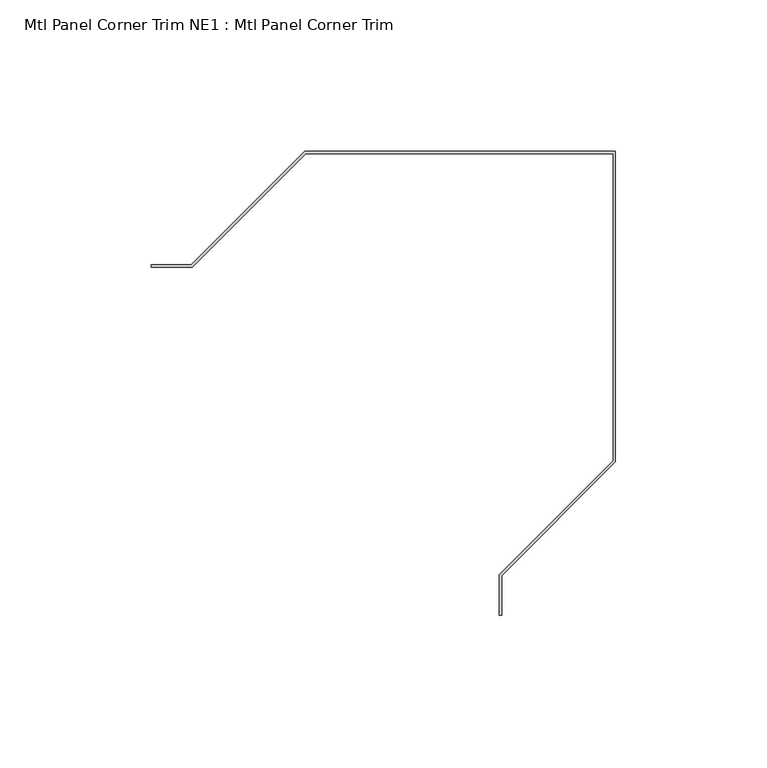
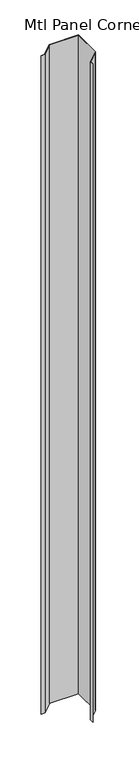
"""IFC4 building model written with IfcOpenShell, lengths in millimetres: proxy geometry, Mtl Panel Corner Trim NE1 : Mtl Panel Corner Trim."""

from ifc_helpers import new_model, si_unit, frame, origin, place, context, project, spatial, polyline, outline, extrude, source, transform, mapped, element, save


def mtl_panel_corner_trim_ne1_mtl_panel_corner_trim_1dc4974f(model_context):
    return source(origin(), model_context, "Body", "SweptSolid", [
        extrude(outline(polyline([(590354.0764739, -531753.7703841), (590354.0764739, -531740.2994038), (590391.6621239, -531702.7137538), (590391.6621239, -531601.1227341), (590290.0711042, -531601.1227341), (590252.5807042, -531638.6131341), (590239.0144739, -531638.6131341), (590239.0144739, -531637.8193841), (590252.2519222, -531637.8193841), (590289.7423222, -531600.3289841), (590392.4558739, -531600.3289841), (590392.4558739, -531703.0425358), (590354.8638739, -531740.6345358), (590354.8638739, -531753.7703841), (590354.0764739, -531753.7703841)])), frame((0.0, 0.0, 6.35), z_axis=(0.0, 0.0, 1.0), x_axis=(1.0, 0.0, 0.0)), (0.0, 0.0, 1.0), 2432.05),
    ])


if __name__ == "__main__":
    model = new_model("IFC4")
    model_context = context("Model", 3, world=origin())
    ifc_project = project(units=[si_unit("LENGTHUNIT", "METRE", prefix="MILLI")], contexts=[model_context])
    site = spatial("IfcSite", under=ifc_project)
    building = spatial("IfcBuilding", under=site)
    placement = place(None, origin())
    mtl_panel_corner_trim_ne1_mtl_panel_corner_trim_shape = mtl_panel_corner_trim_ne1_mtl_panel_corner_trim_1dc4974f(model_context)
    element("IfcBuildingElementProxy", 1, Name="Mtl Panel Corner Trim NE1 : Mtl Panel Corner Trim", ObjectType="Mtl Panel Corner Trim NE1 : Mtl Panel Corner Trim", at=placement, inside=building, context=model_context, shape_type="MappedRepresentation", body=[
        mapped(mtl_panel_corner_trim_ne1_mtl_panel_corner_trim_shape, transform((0.0, 0.0, 0.0), x_axis=(1.0, 0.0, 0.0), y_axis=(0.0, 1.0, 0.0), z_axis=(0.0, 0.0, 1.0))),
    ])
    save(model, "model.ifc")

# Revit data of these elements
# Element 1 (IfcBuildingElementProxy, "Mtl Panel Corner Trim NE1 : Mtl Panel Corner Trim")
#   Materials on its faces: "CORNER TRIM BY MTL PANEL MFR."
# Materials
#   "CORNER TRIM BY MTL PANEL MFR.": class "Generic", colour RGB 239 242 240, transparency 0, Cost = 0
